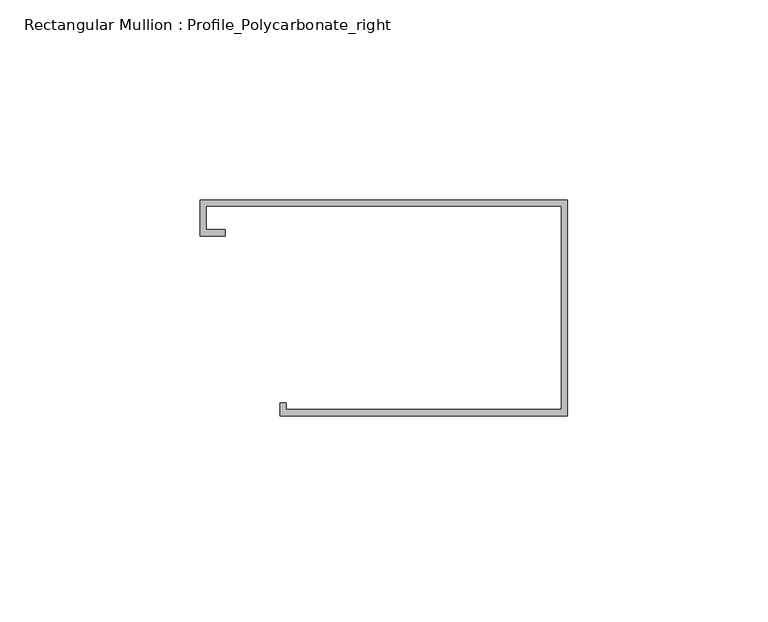
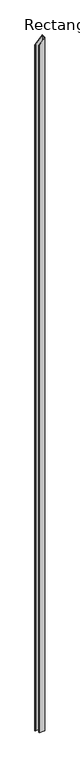
"""IFC4 building model written with IfcOpenShell, lengths in millimetres: member geometry, Rectangular Mullion : Profile_Polycarbonate_right."""

import ifcopenshell
import ifcopenshell.guid

model = None  # the IFC model being written
_history = None  # IfcOwnerHistory: only IFC2X3 demands one
_inside = {}  # id of a spatial element -> (the spatial element, [elements in it])
_under = {}  # id of a project, library or spatial element -> (it, [spatial elements below it])
_declared = {}  # id of a project -> (the project, [libraries it declares])
_typed = {}  # id of a type object -> (the type object, [elements of that type])
_made_of = {}  # id of a material, layer set ... -> (it, [elements and type objects made of it])


def new_model(schema):
    """Start an empty IFC model of exactly this schema.

    Asked for "IFC4X3", IfcOpenShell would pick the latest addendum, in which some entities
    have other attributes; the version numbers below select the first issue.
    IFC2X3 requires an IfcOwnerHistory on every rooted entity: one is made here for all.
    """
    global model, _history
    if schema == "IFC4X3":
        model = ifcopenshell.file(schema_version=(4, 3, 0, 0))
    else:
        model = ifcopenshell.file(schema=schema)
    _inside.clear()
    _under.clear()
    _declared.clear()
    _typed.clear()
    _made_of.clear()
    _history = None
    if model.schema == "IFC2X3":
        org = make("IfcOrganization", Name="unknown")
        user = make(
            "IfcPersonAndOrganization",
            ThePerson=make("IfcPerson", FamilyName="unknown"),
            TheOrganization=org,
        )
        app = make(
            "IfcApplication",
            ApplicationDeveloper=org,
            Version="unknown",
            ApplicationFullName="unknown",
            ApplicationIdentifier="unknown",
        )
        _history = make(
            "IfcOwnerHistory",
            OwningUser=user,
            OwningApplication=app,
            ChangeAction="ADDED",
            CreationDate=0,
        )
    return model


def make(cls, **values):
    """One entity of the class cls with the attributes given. An attribute that is None is left unset."""
    return model.create_entity(
        cls, **{name: value for name, value in values.items() if value is not None}
    )


def rooted(cls, **values):
    """An entity with a GlobalId (a new one), such as an element, a storey or a relation."""
    return make(cls, GlobalId=ifcopenshell.guid.new(), OwnerHistory=_history, **values)


def si_unit(unit_type, name, prefix=None):
    """IfcSIUnit, for example si_unit("LENGTHUNIT", "METRE", prefix="MILLI")."""
    return make("IfcSIUnit", UnitType=unit_type, Prefix=prefix, Name=name)


def assignment(units):
    """IfcUnitAssignment: the units of a project."""
    return None if units is None else make("IfcUnitAssignment", Units=units)


def point(xyz):
    """IfcCartesianPoint."""
    return None if xyz is None else make("IfcCartesianPoint", Coordinates=xyz)


def direction(xyz):
    """IfcDirection."""
    return None if xyz is None else make("IfcDirection", DirectionRatios=xyz)


def frame(location, z_axis=None, x_axis=None):
    """IfcAxis2Placement3D, a coordinate frame: its origin and axes. An axis left out is left unset."""
    return make(
        "IfcAxis2Placement3D",
        Location=point(location),
        Axis=direction(z_axis),
        RefDirection=direction(x_axis),
    )


def origin():
    """The frame at (0, 0, 0) with its axes left unset."""
    return frame((0.0, 0.0, 0.0))


def place(relative_to, where):
    """IfcLocalPlacement: puts the frame where relative to a parent placement (None: the world)."""
    return make(
        "IfcLocalPlacement", PlacementRelTo=relative_to, RelativePlacement=where
    )


def context(
    kind, dimensions, precision=None, world=None, true_north=None, identifier=None
):
    """IfcGeometricRepresentationContext, for example the 3D "Model" context."""
    return make(
        "IfcGeometricRepresentationContext",
        ContextIdentifier=identifier,
        ContextType=kind,
        CoordinateSpaceDimension=dimensions,
        Precision=precision,
        WorldCoordinateSystem=world,
        TrueNorth=true_north,
    )


def project(units=None, contexts=None):
    """IfcProject with its units and contexts."""
    return rooted(
        "IfcProject",
        Name="project",
        RepresentationContexts=contexts,
        UnitsInContext=assignment(units),
    )


def spatial(cls, under=None, at=None, **own):
    """A site, building, storey or space (cls), placed at a placement, below another one or the project."""
    s = rooted(cls, ObjectPlacement=at, **own)
    if under is not None:
        _under.setdefault(under.id(), (under, []))[1].append(s)
    return s


def faces_of(points, faces, orient=None, outer=None):
    """IfcFace entities. A face is a list of loops; a loop is a list of indices into points, from 0.

    orient and outer hold one flag for each loop. By default every Orientation is true, the
    first loop of a face is its IfcFaceOuterBound and the others are IfcFaceBound.
    """
    made = []
    for i, loops in enumerate(faces):
        bounds = []
        for j, loop in enumerate(loops):
            is_outer = j == 0 if outer is None else outer[i][j]
            bounds.append(
                make(
                    "IfcFaceOuterBound" if is_outer else "IfcFaceBound",
                    Bound=make("IfcPolyLoop", Polygon=[points[k] for k in loop]),
                    Orientation=True if orient is None else orient[i][j],
                )
            )
        made.append(make("IfcFace", Bounds=bounds))
    return made


def faceted_brep(points, faces, orient=None, outer=None, voids=None):
    """IfcFacetedBrep: a solid bounded by flat faces; with voids (closed shells), ...WithVoids."""
    shared = [point(p) for p in points]
    hull = make("IfcClosedShell", CfsFaces=faces_of(shared, faces, orient, outer))
    if voids is None:
        return make("IfcFacetedBrep", Outer=hull)
    return make(
        "IfcFacetedBrepWithVoids",
        Outer=hull,
        Voids=[
            make(cls, CfsFaces=faces_of(shared, fs, o, b)) for cls, fs, o, b in voids
        ],
    )


def shape(context_of_items, identifier, shape_type, items):
    """IfcShapeRepresentation: the items that make up one representation, for example the "Body"."""
    return make(
        "IfcShapeRepresentation",
        ContextOfItems=context_of_items,
        RepresentationIdentifier=identifier,
        RepresentationType=shape_type,
        Items=items,
    )


def source(mapping_origin, context_of_items, identifier, shape_type, items):
    """IfcRepresentationMap: a shape defined once, which mapped items show again and again."""
    return make(
        "IfcRepresentationMap",
        MappingOrigin=mapping_origin,
        MappedRepresentation=shape(context_of_items, identifier, shape_type, items),
    )


def transform(
    local_origin,
    x_axis=None,
    y_axis=None,
    z_axis=None,
    scale=None,
    scale2=None,
    scale3=None,
    uniform=True,
):
    """IfcCartesianTransformationOperator3D, or its non-uniform kind. x_axis, y_axis, z_axis: its Axis1, 2, 3."""
    if uniform:
        return make(
            "IfcCartesianTransformationOperator3D",
            Axis1=direction(x_axis),
            Axis2=direction(y_axis),
            LocalOrigin=point(local_origin),
            Scale=scale,
            Axis3=direction(z_axis),
        )
    return make(
        "IfcCartesianTransformationOperator3DnonUniform",
        Axis1=direction(x_axis),
        Axis2=direction(y_axis),
        LocalOrigin=point(local_origin),
        Scale=scale,
        Axis3=direction(z_axis),
        Scale2=scale2,
        Scale3=scale3,
    )


def mapped(mapping_source, mapping_target):
    """IfcMappedItem: shows the shape of a source again, moved by a transform."""
    return make(
        "IfcMappedItem", MappingSource=mapping_source, MappingTarget=mapping_target
    )


def made_of(thing, what):
    """Note that an element or type object is made of a material, layer set ...; save() writes the relation."""
    if what is not None:
        _made_of.setdefault(what.id(), (what, []))[1].append(thing)
    return thing


def element(
    cls,
    number,
    at=None,
    inside=None,
    cuts=None,
    type_object=None,
    material=None,
    context=None,
    identifier="Body",
    shape_type=None,
    held_by="IfcProductDefinitionShape",
    body=None,
    shapes=None,
    **own,
):
    """One element of the class cls, such as IfcWall. Its Tag is "e" and its number.

    at: its placement. inside: the storey or other place that contains it. cuts: it is an
    opening in that element (IfcRelVoidsElement). A single representation is given by context,
    identifier, shape_type and body (its items); several are given by shapes. held_by: the class
    of the entity that holds the representations. save() writes the other relations.
    """
    e = rooted(cls, Tag="e%d" % number, ObjectPlacement=at, **own)
    if body is not None:
        shapes = [shape(context, identifier, shape_type, body)]
    if shapes is not None:
        e.Representation = make(held_by, Representations=shapes)
    if inside is not None:
        _inside.setdefault(inside.id(), (inside, []))[1].append(e)
    if cuts is not None:
        rooted(
            "IfcRelVoidsElement", RelatingBuildingElement=cuts, RelatedOpeningElement=e
        )
    if type_object is not None:
        _typed.setdefault(type_object.id(), (type_object, []))[1].append(e)
    return made_of(e, material)


def aggregate(whole, parts):
    """IfcRelAggregates: a whole, such as a stair, and the parts it consists of."""
    return rooted("IfcRelAggregates", RelatingObject=whole, RelatedObjects=parts)


def save(model, path):
    """Write the relations noted so far, then the file.

    IfcRelAggregates (storeys below a building ...), IfcRelContainedInSpatialStructure (elements
    in a storey), IfcRelDefinesByType, IfcRelAssociatesMaterial and IfcRelDeclares: one each for
    every whole, place, type object, material and project.
    """
    for whole, parts in _under.values():
        aggregate(whole, parts)
    for where, things in _inside.values():
        rooted(
            "IfcRelContainedInSpatialStructure",
            RelatedElements=things,
            RelatingStructure=where,
        )
    for kind, things in _typed.values():
        rooted("IfcRelDefinesByType", RelatedObjects=things, RelatingType=kind)
    for what, things in _made_of.values():
        rooted("IfcRelAssociatesMaterial", RelatedObjects=things, RelatingMaterial=what)
    for by, libraries in _declared.values():
        rooted("IfcRelDeclares", RelatingContext=by, RelatedDefinitions=libraries)
    model.write(path)


def rectangular_mullion_profile_polycarbonate_right_2daa0c8d(model_context):
    return source(origin(), model_context, "Body", "Brep", [
        faceted_brep([(0.0, 28.984575, -8947.4969961), (0.0, -25.015825, -8947.4969961), (-71.9836, -25.015825, -8947.4969961), (-71.9836, -21.840825, -8947.4969961), (-70.3961, -21.840825, -8947.4969961), (-70.3961, -23.428325, -8947.4969961), (-1.5875, -23.428325, -8947.4969961), (-1.5875, 27.397075, -8947.4969961), (-90.4113, 27.397075, -8947.4969961), (-90.4113, 21.580475, -8947.4969961), (-85.6488, 21.580475, -8947.4969961), (-85.6488, 19.992975, -8947.4969961), (-91.9988, 19.992975, -8947.4969961), (-91.9988, 28.984575, -8947.4969961), (-91.9988, 28.984575, -95.9119088), (0.0, 28.984575, 0.0), (-91.9988, 19.992975, -95.9119088), (-85.6488, 19.992975, -89.2918157), (-85.6488, 21.580475, -89.2918157), (-90.4113, 21.580475, -94.2568855), (-90.4113, 27.397075, -94.2568855), (-1.5875, 27.397075, -1.6550233), (-1.5875, -23.428325, -1.6550233), (-70.3961, -23.428325, -73.3903521), (-70.3961, -21.840825, -73.3903521), (-71.9836, -21.840825, -75.0453753), (-71.9836, -25.015825, -75.0453753), (0.0, -25.015825, 0.0)], [[[0, 1, 2, 3, 4, 5, 6, 7, 8, 9, 10, 11, 12, 13]], [[14, 15, 0, 13]], [[16, 14, 13, 12]], [[17, 16, 12, 11]], [[18, 17, 11, 10]], [[19, 18, 10, 9]], [[20, 19, 9, 8]], [[21, 20, 8, 7]], [[22, 21, 7, 6]], [[23, 22, 6, 5]], [[24, 23, 5, 4]], [[25, 24, 4, 3]], [[26, 25, 3, 2]], [[27, 26, 2, 1]], [[15, 27, 1, 0]], [[15, 14, 16, 17, 18, 19, 20, 21, 22, 23, 24, 25, 26, 27]]]),
    ])


if __name__ == "__main__":
    model = new_model("IFC4")
    model_context = context("Model", 3, world=origin())
    ifc_project = project(units=[si_unit("LENGTHUNIT", "METRE", prefix="MILLI")], contexts=[model_context])
    site = spatial("IfcSite", under=ifc_project)
    building = spatial("IfcBuilding", under=site)
    placement = place(None, origin())
    rectangular_mullion_profile_polycarbonate_right_shape = rectangular_mullion_profile_polycarbonate_right_2daa0c8d(model_context)
    element("IfcMember", 1, ObjectType="Rectangular Mullion : Profile_Polycarbonate_right", at=placement, inside=building, context=model_context, shape_type="MappedRepresentation", body=[
        mapped(rectangular_mullion_profile_polycarbonate_right_shape, transform((0.0, 0.0, 0.0), x_axis=(1.0, 0.0, 0.0), y_axis=(0.0, 1.0, 0.0), z_axis=(0.0, 0.0, 1.0))),
    ])
    save(model, "model.ifc")

# Revit data of these elements
# Type "Rectangular Mullion : Profile_Polycarbonate_right"
#   built-in parameter 1007322 = 0.177167 (stored number, unit not read)
#   built-in parameter 1007321 = 0 (stored number, unit not read)
#   built-in parameter 1007320 = 0.00520833 (stored number, unit not read)
